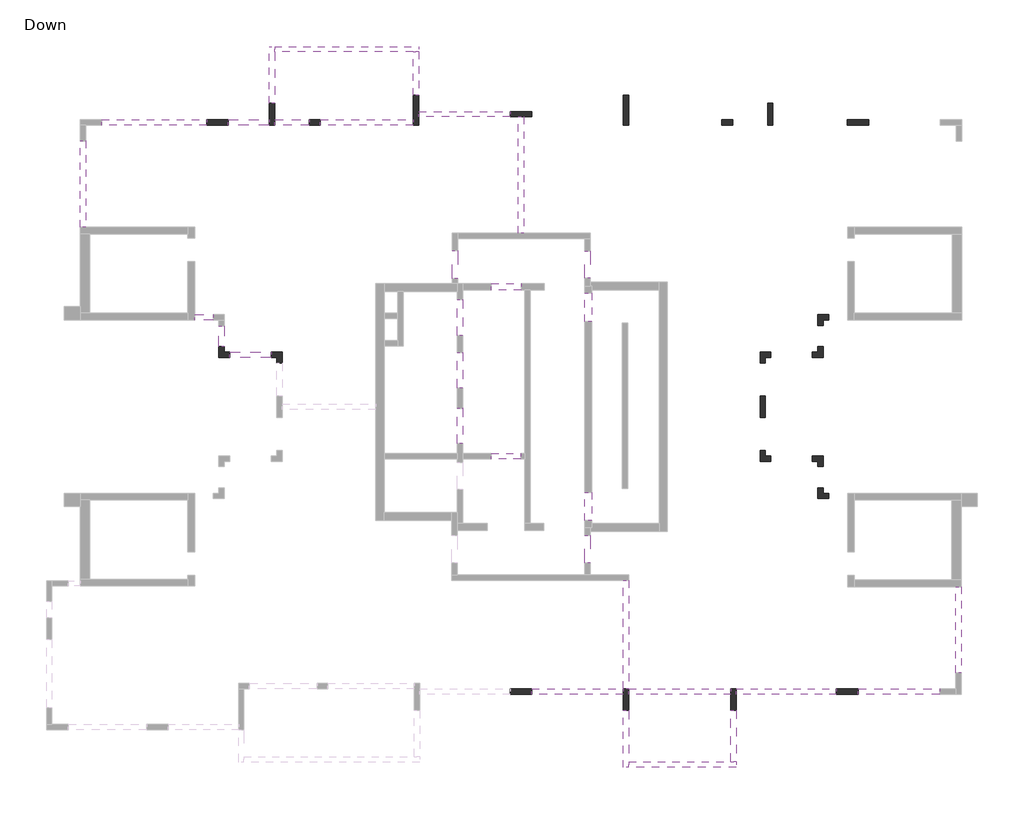
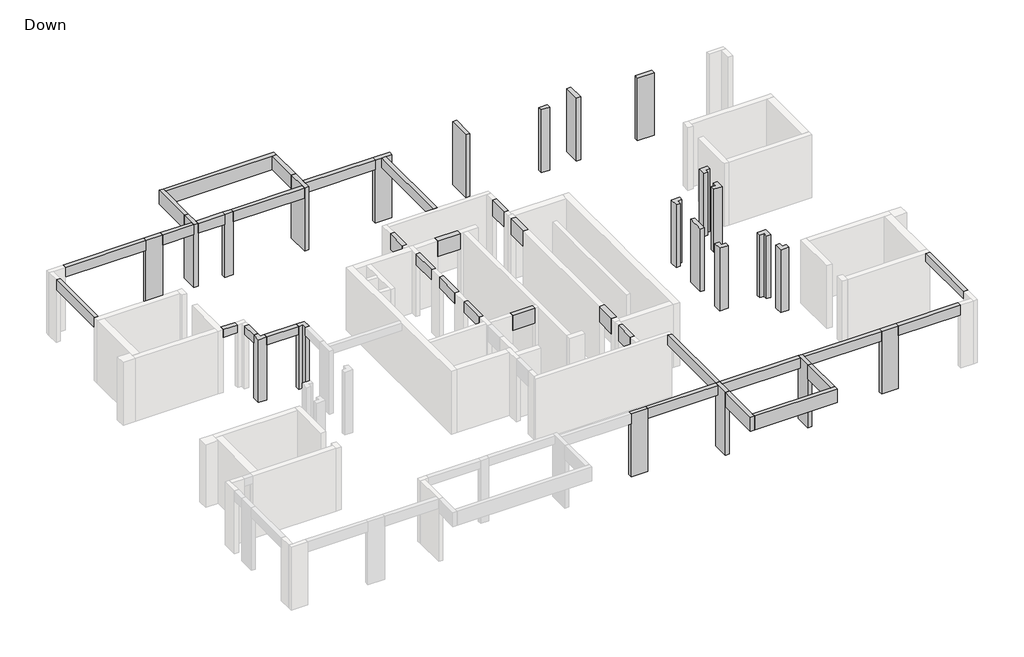
# One storey, part 3 of 3: 32 beams, 22 columns.
"""IFC4 building model written with IfcOpenShell, lengths in millimetres."""

from ifc_helpers import new_model, si_unit, frame, origin, origin_with_axes, place, context, project, spatial, polyline, outline, extrude, faceted_brep, element, save

model = new_model("IFC4")

# Units and contexts
model_context = context("Model", 3, world=origin())
ifc_project = project(units=[si_unit("LENGTHUNIT", "METRE", prefix="MILLI")], contexts=[model_context])

# Site, building, storey
site = spatial("IfcSite", under=ifc_project)
building = spatial("IfcBuilding", under=site)
storey = spatial("IfcBuildingStorey", under=building, Name="Down", Elevation=0.0)

# Beams
placement = place(None, origin())
element("IfcBeam", 1, ObjectType="Concrete Rectengular Beam : 20/40", at=placement, inside=storey, context=model_context, shape_type="Brep", body=[
    faceted_brep([(-11929.8186713, 1705.2784849, 3200.0), (-11929.8186713, 1505.2784849, 3200.0), (-11231.2965038, 1505.2784849, 3200.0), (-11231.2965038, 1705.2784849, 3200.0), (-11231.2965038, 1705.2784849, 3020.0), (-11231.2965038, 1705.2784849, 2800.0), (-11929.8186713, 1705.2784849, 2800.0), (-11929.8186713, 1705.2784849, 3020.0), (-11929.8186713, 1505.2784849, 2800.0), (-11231.2965038, 1505.2784849, 2800.0)], [[[0, 1, 2, 3]], [[0, 3, 4, 5, 6, 7]], [[8, 6, 5, 9]], [[1, 8, 9, 2]], [[1, 0, 7, 6, 8]], [[3, 2, 9, 5, 4]]]),
])
element("IfcBeam", 2, ObjectType="Concrete Rectengular Beam : 20/40", at=placement, inside=storey, context=model_context, shape_type="Brep", body=[
    faceted_brep([(-10831.2965038, 1285.2784849, 3200.0), (-11031.2965038, 1285.2784849, 3200.0), (-11031.2965038, 525.2784849, 3200.0), (-10831.2965038, 525.2784849, 3200.0), (-11031.2965038, 1285.2784849, 2800.0), (-11031.2965038, 525.2784849, 2800.0), (-10831.2965038, 1285.2784849, 2800.0), (-10831.2965038, 525.2784849, 2800.0), (-10831.2965038, 1285.2784849, 3020.0)], [[[0, 1, 2, 3]], [[1, 4, 5, 2]], [[4, 6, 7, 5]], [[6, 8, 0, 3, 7]], [[1, 0, 8, 6, 4]], [[3, 2, 5, 7]]]),
])
element("IfcBeam", 3, ObjectType="Concrete Rectengular Beam : 20/40", at=placement, inside=storey, context=model_context, shape_type="SweptSolid", body=[
    extrude(outline(polyline([(-10631.2965038, 125.2784849), (-10631.2965038, 325.2784849), (-9097.9894431, 325.2784849), (-9097.9894431, 125.2784849), (-10631.2965038, 125.2784849)])), frame((0.0, 0.0, 2800.0), z_axis=(0.0, 0.0, 1.0), x_axis=(1.0, 0.0, 0.0)), (0.0, 0.0, 1.0), 400.0),
])
element("IfcBeam", 4, ObjectType="Concrete Rectengular Beam : 20/40", at=placement, inside=storey, context=model_context, shape_type="Brep", body=[
    faceted_brep([(16390.4478267, -8347.5852261, 3200.0), (16190.4478267, -8347.5852261, 3200.0), (16190.4478267, -11524.2691374, 3200.0), (16390.4478267, -11524.2691374, 3200.0), (16390.4478267, -8347.5852261, 2800.0), (16390.4478267, -11524.2691374, 2800.0), (16190.4478267, -8347.5852261, 2800.0), (16190.4478267, -11524.2691374, 2800.0), (16190.4478267, -8347.5852261, 3020.0)], [[[0, 1, 2, 3]], [[4, 0, 3, 5]], [[6, 4, 5, 7]], [[1, 8, 6, 7, 2]], [[1, 0, 4, 6, 8]], [[3, 2, 7, 5]]]),
])
element("IfcBeam", 5, ObjectType="Concrete Rectengular Beam : 20/50", at=placement, inside=storey, context=model_context, shape_type="Brep", body=[
    faceted_brep([(-3849.7912929, 8714.1448811, 3200.0), (-3849.7912929, 8914.1448811, 3200.0), (-7285.8677257, 8914.1448811, 3200.0), (-7285.8677257, 8714.1448811, 3200.0), (-3849.7912929, 8914.1448811, 3020.0), (-3849.7912929, 8914.1448811, 2700.0), (-7285.8677257, 8914.1448811, 2700.0), (-3849.7912929, 8714.1448811, 2700.0), (-7285.8677257, 8714.1448811, 2700.0), (-7285.8677257, 8714.1448811, 3020.0), (-3849.7912929, 8714.1448811, 3020.0)], [[[0, 1, 2, 3]], [[1, 4, 5, 6, 2]], [[5, 7, 8, 6]], [[0, 3, 9, 8, 7, 10]], [[1, 0, 10, 7, 5, 4]], [[3, 2, 6, 8, 9]]]),
])
element("IfcBeam", 6, ObjectType="Concrete Rectengular Beam : 20/50", at=placement, inside=storey, context=model_context, shape_type="Brep", body=[
    faceted_brep([(-7685.8677257, 8714.1448811, 3200.0), (-7685.8677257, 8914.1448811, 3200.0), (-8975.1176117, 8914.1448811, 3200.0), (-8975.1176117, 8714.1448811, 3200.0), (-7685.8677257, 8914.1448811, 2700.0), (-8975.1176117, 8914.1448811, 2700.0), (-8975.1176117, 8914.1448811, 3020.0), (-7685.8677257, 8714.1448811, 2700.0), (-8975.1176117, 8714.1448811, 2700.0), (-8975.1176117, 8714.1448811, 3020.0), (-7685.8677257, 8714.1448811, 3020.0)], [[[0, 1, 2, 3]], [[1, 4, 5, 6, 2]], [[4, 7, 8, 5]], [[0, 3, 9, 8, 7, 10]], [[1, 0, 10, 7, 4]], [[3, 2, 6, 5, 8, 9]]]),
])
element("IfcBeam", 7, ObjectType="Concrete Rectengular Beam : 20/50", at=placement, inside=storey, context=model_context, shape_type="Brep", body=[
    faceted_brep([(-9175.1176117, 8714.1448811, 3200.0), (-9175.1176117, 8914.1448811, 3200.0), (-10684.1955166, 8914.1448811, 3200.0), (-10684.1955166, 8714.1448811, 3200.0), (-9175.1176117, 8914.1448811, 2700.0), (-10684.1955166, 8914.1448811, 2700.0), (-9175.1176117, 8714.1448811, 2700.0), (-10684.1955166, 8714.1448811, 2700.0), (-10684.1955166, 8714.1448811, 3020.0), (-9175.1176117, 8714.1448811, 3020.0)], [[[0, 1, 2, 3]], [[1, 4, 5, 2]], [[4, 6, 7, 5]], [[0, 3, 8, 7, 6, 9]], [[1, 0, 9, 6, 4]], [[3, 2, 5, 7, 8]]]),
])
element("IfcBeam", 8, ObjectType="Concrete Rectengular Beam : 20/50", at=placement, inside=storey, context=model_context, shape_type="Brep", body=[
    faceted_brep([(-11484.1955166, 8714.1448811, 3200.0), (-11484.1955166, 8914.1448811, 3200.0), (-15359.5625137, 8914.1448811, 3200.0), (-15359.5625137, 8714.1448811, 3200.0), (-11484.1955166, 8914.1448811, 2700.0), (-15359.5625137, 8914.1448811, 2700.0), (-11484.1955166, 8714.1448811, 2700.0), (-15359.5625137, 8714.1448811, 2700.0), (-15359.5625137, 8714.1448811, 3020.0), (-11484.1955166, 8714.1448811, 3020.0)], [[[0, 1, 2, 3]], [[1, 4, 5, 2]], [[4, 6, 7, 5]], [[0, 3, 8, 7, 6, 9]], [[1, 0, 9, 6, 4]], [[3, 2, 5, 7, 8]]]),
])
element("IfcBeam", 9, ObjectType="Concrete Rectengular Beam : 20/50", at=placement, inside=storey, context=model_context, shape_type="Brep", body=[
    faceted_brep([(-15952.3851738, 8125.9123109, 3200.0), (-16152.3851738, 8125.9123109, 3200.0), (-16152.3851738, 4939.6791417, 3200.0), (-15952.3851738, 4939.6791417, 3200.0), (-16152.3851738, 8125.9123109, 2700.0), (-16152.3851738, 4939.6791417, 2700.0), (-15952.3851738, 8125.9123109, 2700.0), (-15952.3851738, 4939.6791417, 2700.0), (-15952.3851738, 4939.6791417, 3020.0)], [[[0, 1, 2, 3]], [[1, 4, 5, 2]], [[4, 6, 7, 5]], [[6, 0, 3, 8, 7]], [[1, 0, 6, 4]], [[3, 2, 5, 7, 8]]]),
])
element("IfcBeam", 10, ObjectType="Concrete Rectengular Beam : 20/50", at=placement, inside=storey, context=model_context, shape_type="Brep", body=[
    faceted_brep([(-3649.7912929, 9214.1448811, 3200.0), (-3649.7912929, 9014.1448811, 3200.0), (-270.9686735, 9014.1448811, 3200.0), (-270.9686735, 9214.1448811, 3200.0), (-3649.7912929, 9214.1448811, 2700.0), (-270.9686735, 9214.1448811, 2700.0), (-3649.7912929, 9014.1448811, 2700.0), (-270.9686735, 9014.1448811, 2700.0), (-3649.7912929, 9014.1448811, 3020.0)], [[[0, 1, 2, 3]], [[4, 0, 3, 5]], [[6, 4, 5, 7]], [[1, 8, 6, 7, 2]], [[1, 0, 4, 6, 8]], [[3, 2, 7, 5]]]),
])
element("IfcBeam", 11, ObjectType="Concrete Rectengular Beam : 20/50", at=placement, inside=storey, context=model_context, shape_type="Brep", body=[
    faceted_brep([(229.0313265, 9014.1448811, 3200.0), (29.0313265, 9014.1448811, 3200.0), (29.0313265, 4709.9784533, 3200.0), (229.0313265, 4709.9784533, 3200.0), (29.0313265, 9014.1448811, 3020.0), (29.0313265, 9014.1448811, 2700.0), (29.0313265, 4709.9784533, 2700.0), (29.0313265, 4709.9784533, 3020.0), (229.0313265, 9014.1448811, 2700.0), (229.0313265, 4709.9784533, 2700.0), (229.0313265, 9014.1448811, 3020.0), (229.0313265, 4709.9784533, 3020.0)], [[[0, 1, 2, 3]], [[1, 4, 5, 6, 7, 2]], [[5, 8, 9, 6]], [[8, 10, 0, 3, 11, 9]], [[5, 4, 1, 0, 10, 8]], [[3, 2, 7, 6, 9, 11]]]),
])
element("IfcBeam", 12, ObjectType="Concrete Rectengular Beam : 20/50", at=placement, inside=storey, context=model_context, shape_type="SweptSolid", body=[
    extrude(outline(polyline([(12576.1675255, -12324.2691374), (12576.1675255, -12124.2691374), (15592.9268131, -12124.2691374), (15592.9268131, -12324.2691374), (12576.1675255, -12324.2691374)])), frame((0.0, 0.0, 2700.0), z_axis=(0.0, 0.0, 1.0), x_axis=(1.0, 0.0, 0.0)), (0.0, 0.0, 1.0), 500.0),
])
element("IfcBeam", 13, ObjectType="Concrete Rectengular Beam : 20/50", at=placement, inside=storey, context=model_context, shape_type="Brep", body=[
    faceted_brep([(11776.1675255, -12324.2691374, 3200.0), (11776.1675255, -12124.2691374, 3200.0), (8077.9664013, -12124.2691374, 3200.0), (8077.9664013, -12324.2691374, 3200.0), (11776.1675255, -12124.2691374, 2700.0), (8077.9664013, -12124.2691374, 2700.0), (8077.9664013, -12124.2691374, 3020.0), (11776.1675255, -12324.2691374, 2700.0), (8077.9664013, -12324.2691374, 2700.0)], [[[0, 1, 2, 3]], [[1, 4, 5, 6, 2]], [[4, 7, 8, 5]], [[7, 0, 3, 8]], [[1, 0, 7, 4]], [[3, 2, 6, 5, 8]]]),
])
element("IfcBeam", 14, ObjectType="Concrete Rectengular Beam : 20/50", at=placement, inside=storey, context=model_context, shape_type="Brep", body=[
    faceted_brep([(7877.9664013, -12324.2691374, 3200.0), (7877.9664013, -12124.2691374, 3200.0), (4107.8539459, -12124.2691374, 3200.0), (4107.8539459, -12324.2691374, 3200.0), (7877.9664013, -12124.2691374, 3020.0), (7877.9664013, -12124.2691374, 2700.0), (4107.8539459, -12124.2691374, 2700.0), (4107.8539459, -12124.2691374, 3020.0), (7877.9664013, -12324.2691374, 2700.0), (4107.8539459, -12324.2691374, 2700.0), (7877.9664013, -12324.2691374, 3020.0), (4107.8539459, -12324.2691374, 3020.0)], [[[0, 1, 2, 3]], [[1, 4, 5, 6, 7, 2]], [[5, 8, 9, 6]], [[8, 10, 0, 3, 11, 9]], [[1, 0, 10, 8, 5, 4]], [[3, 2, 7, 6, 9, 11]]]),
])
element("IfcBeam", 15, ObjectType="Concrete Rectengular Beam : 20/50", at=placement, inside=storey, context=model_context, shape_type="Brep", body=[
    faceted_brep([(3907.8539459, -12324.2691374, 3200.0), (3907.8539459, -12124.2691374, 3200.0), (529.0313265, -12124.2691374, 3200.0), (529.0313265, -12324.2691374, 3200.0), (3907.8539459, -12124.2691374, 3020.0), (3907.8539459, -12124.2691374, 2700.0), (529.0313265, -12124.2691374, 2700.0), (529.0313265, -12124.2691374, 3020.0), (3907.8539459, -12324.2691374, 2700.0), (529.0313265, -12324.2691374, 2700.0)], [[[0, 1, 2, 3]], [[2, 1, 4, 5, 6, 7]], [[5, 8, 9, 6]], [[8, 0, 3, 9]], [[1, 0, 8, 5, 4]], [[3, 2, 7, 6, 9]]]),
])
element("IfcBeam", 16, ObjectType="Concrete Rectengular Beam : 20/50", at=placement, inside=storey, context=model_context, shape_type="Brep", body=[
    faceted_brep([(3907.8539459, -12124.2691374, 3200.0), (4107.8539459, -12124.2691374, 3200.0), (4107.8539459, -8111.1752209, 3200.0), (3907.8539459, -8111.1752209, 3200.0), (4107.8539459, -12124.2691374, 3020.0), (4107.8539459, -12124.2691374, 2700.0), (4107.8539459, -8111.1752209, 2700.0), (3907.8539459, -12124.2691374, 2700.0), (3907.8539459, -8111.1752209, 2700.0), (3907.8539459, -12124.2691374, 3020.0), (3907.8539459, -8111.1752209, 3020.0)], [[[0, 1, 2, 3]], [[1, 4, 5, 6, 2]], [[5, 7, 8, 6]], [[7, 9, 0, 3, 10, 8]], [[0, 9, 7, 5, 4, 1]], [[3, 2, 6, 8, 10]]]),
])
element("IfcBeam", 17, ObjectType="Concrete Rectengular Beam : 20/53", at=placement, inside=storey, context=model_context, shape_type="SweptSolid", body=[
    extrude(outline(polyline([(3200.0, -2227.8189264), (2670.0, -2227.8189264), (2670.0, -2027.8189264), (3020.0, -2027.8189264), (3020.0, -2032.8189264), (3200.0, -2032.8189264), (3200.0, -2227.8189264)])), frame((0.0, 933.8247791, 0.0), z_axis=(0.0, 1.0, 0.0), x_axis=(0.0, 0.0, 1.0)), (0.0, 0.0, 1.0), 1325.0),
])
element("IfcBeam", 18, ObjectType="Concrete Rectengular Beam : 20/53", at=placement, inside=storey, context=model_context, shape_type="SweptSolid", body=[
    extrude(outline(polyline([(3200.0, -2227.8189264), (2670.0, -2227.8189264), (2670.0, -2027.8189264), (3020.0, -2027.8189264), (3020.0, -2032.8189264), (3200.0, -2032.8189264), (3200.0, -2227.8189264)])), frame((0.0, -1013.9530422, 0.0), z_axis=(0.0, 1.0, 0.0), x_axis=(0.0, 0.0, 1.0)), (0.0, 0.0, 1.0), 1327.7778213),
])
element("IfcBeam", 19, ObjectType="Concrete Rectengular Beam : 20/53", at=placement, inside=storey, context=model_context, shape_type="SweptSolid", body=[
    extrude(outline(polyline([(3200.0, -2227.8189264), (2670.0, -2227.8189264), (2670.0, -2027.8189264), (3020.0, -2027.8189264), (3020.0, -2032.8189264), (3200.0, -2032.8189264), (3200.0, -2227.8189264)])), frame((0.0, -3053.9530422, 0.0), z_axis=(0.0, 1.0, 0.0), x_axis=(0.0, 0.0, 1.0)), (0.0, 0.0, 1.0), 1300.0),
])
element("IfcBeam", 20, ObjectType="Concrete Rectengular Beam : 20/70", at=placement, inside=storey, context=model_context, shape_type="Brep", body=[
    faceted_brep([(-8975.1176117, 11614.1448811, 3200.0), (-9175.1176117, 11614.1448811, 3200.0), (-9175.1176117, 9514.1448811, 3200.0), (-8975.1176117, 9514.1448811, 3200.0), (-8975.1176117, 11414.1448811, 3200.0), (-8975.1176117, 11614.1448811, 2500.0), (-8975.1176117, 9514.1448811, 2500.0), (-8975.1176117, 11414.1448811, 2500.0), (-9175.1176117, 11614.1448811, 2500.0), (-9175.1176117, 9514.1448811, 2500.0)], [[[0, 1, 2, 3, 4]], [[5, 0, 4, 3, 6, 7]], [[8, 5, 7, 6, 9]], [[1, 8, 9, 2]], [[3, 2, 9, 6]], [[1, 0, 5, 8]]]),
])
element("IfcBeam", 21, ObjectType="Concrete Rectengular Beam : 20/70", at=placement, inside=storey, context=model_context, shape_type="Brep", body=[
    faceted_brep([(-3649.7912929, 11414.1448811, 3200.0), (-3649.7912929, 11614.1448811, 3200.0), (-8975.1176117, 11614.1448811, 3200.0), (-8975.1176117, 11414.1448811, 3200.0), (-3849.7912929, 11414.1448811, 3200.0), (-3649.7912929, 11414.1448811, 2500.0), (-8975.1176117, 11414.1448811, 3020.0), (-8975.1176117, 11414.1448811, 2500.0), (-3849.7912929, 11414.1448811, 2500.0), (-3649.7912929, 11614.1448811, 2500.0), (-8975.1176117, 11614.1448811, 2500.0)], [[[0, 1, 2, 3, 4]], [[5, 0, 4, 3, 6, 7, 8]], [[9, 5, 8, 7, 10]], [[1, 9, 10, 2]], [[3, 2, 10, 7, 6]], [[1, 0, 5, 9]]]),
])
element("IfcBeam", 22, ObjectType="Concrete Rectengular Beam : 20/70", at=placement, inside=storey, context=model_context, shape_type="Brep", body=[
    faceted_brep([(-3849.7912929, 9814.1448811, 3200.0), (-3649.7912929, 9814.1448811, 3200.0), (-3649.7912929, 11414.1448811, 3200.0), (-3849.7912929, 11414.1448811, 3200.0), (-3849.7912929, 9814.1448811, 2500.0), (-3849.7912929, 11414.1448811, 3020.0), (-3849.7912929, 11414.1448811, 2500.0), (-3649.7912929, 9814.1448811, 2500.0), (-3649.7912929, 11414.1448811, 2500.0)], [[[0, 1, 2, 3]], [[4, 0, 3, 5, 6]], [[7, 4, 6, 8]], [[1, 7, 8, 2]], [[1, 0, 4, 7]], [[3, 2, 8, 6, 5]]]),
])
element("IfcBeam", 23, ObjectType="Concrete Rectengular Beam : 20/70", at=placement, inside=storey, context=model_context, shape_type="Brep", body=[
    faceted_brep([(3907.8539459, -15024.2691374, 3200.0), (4107.8539459, -15024.2691374, 3200.0), (4107.8539459, -14824.2691374, 3200.0), (4107.8539459, -12924.2691374, 3200.0), (3907.8539459, -12924.2691374, 3200.0), (3907.8539459, -15024.2691374, 2500.0), (3907.8539459, -12924.2691374, 2500.0), (4107.8539459, -15024.2691374, 2500.0), (4107.8539459, -12924.2691374, 2500.0), (4107.8539459, -14824.2691374, 2500.0)], [[[0, 1, 2, 3, 4]], [[5, 0, 4, 6]], [[7, 5, 6, 8, 9]], [[1, 7, 9, 8, 3, 2]], [[4, 3, 8, 6]], [[1, 0, 5, 7]]]),
])
element("IfcBeam", 24, ObjectType="Concrete Rectengular Beam : 20/70", at=placement, inside=storey, context=model_context, shape_type="Brep", body=[
    faceted_brep([(8077.9664013, -15024.2691374, 3200.0), (8077.9664013, -14824.2691374, 3200.0), (7877.9664013, -14824.2691374, 3200.0), (4107.8539459, -14824.2691374, 3200.0), (4107.8539459, -15024.2691374, 3200.0), (8077.9664013, -15024.2691374, 2500.0), (4107.8539459, -15024.2691374, 2500.0), (8077.9664013, -14824.2691374, 2500.0), (4107.8539459, -14824.2691374, 2500.0), (7877.9664013, -14824.2691374, 2500.0), (4107.8539459, -14824.2691374, 3020.0)], [[[0, 1, 2, 3, 4]], [[5, 0, 4, 6]], [[7, 5, 6, 8, 9]], [[1, 7, 9, 8, 10, 3, 2]], [[4, 3, 10, 8, 6]], [[1, 0, 5, 7]]]),
])
element("IfcBeam", 25, ObjectType="Concrete Rectengular Beam : 20/70", at=placement, inside=storey, context=model_context, shape_type="Brep", body=[
    faceted_brep([(8077.9664013, -12920.4851141, 3200.0), (7877.9664013, -12920.4851141, 3200.0), (7877.9664013, -14824.2691374, 3200.0), (8077.9664013, -14824.2691374, 3200.0), (8077.9664013, -12920.4851141, 2500.0), (8077.9664013, -14824.2691374, 2500.0), (7877.9664013, -12920.4851141, 2500.0), (7877.9664013, -14824.2691374, 2500.0), (7877.9664013, -14824.2691374, 3020.0)], [[[0, 1, 2, 3]], [[4, 0, 3, 5]], [[6, 4, 5, 7]], [[1, 6, 7, 8, 2]], [[1, 0, 4, 6]], [[3, 2, 8, 7, 5]]]),
])
element("IfcBeam", 26, ObjectType="Concrete Rectengular Beam : 20/78", at=placement, inside=storey, context=model_context, shape_type="Brep", body=[
    faceted_brep([(-2415.274667, 3043.8247791, 3200.0), (-2215.274667, 3043.8247791, 3200.0), (-2215.274667, 4069.9784533, 3200.0), (-2415.274667, 4069.9784533, 3200.0), (-2215.274667, 3043.8247791, 3020.0), (-2215.274667, 3043.8247791, 2420.0), (-2215.274667, 4069.9784533, 2420.0), (-2215.274667, 4069.9784533, 3020.0), (-2415.274667, 3043.8247791, 2420.0), (-2415.274667, 4069.9784533, 2420.0), (-2415.274667, 4069.9784533, 3020.0), (-2415.274667, 3043.8247791, 3020.0)], [[[0, 1, 2, 3]], [[2, 1, 4, 5, 6, 7]], [[5, 8, 9, 6]], [[0, 3, 10, 9, 8, 11]], [[1, 0, 11, 8, 5, 4]], [[3, 2, 7, 6, 9, 10]]]),
])
element("IfcBeam", 27, ObjectType="Concrete Rectengular Beam : 20/78", at=placement, inside=storey, context=model_context, shape_type="SweptSolid", body=[
    extrude(outline(polyline([(2484.725333, 4049.9784533), (2684.725333, 4049.9784533), (2684.725333, 3056.2932633), (2484.725333, 3056.2932633), (2484.725333, 4049.9784533)])), frame((0.0, 0.0, 2420.0), z_axis=(0.0, 0.0, 1.0), x_axis=(1.0, 0.0, 0.0)), (0.0, 0.0, 1.0), 780.0),
])
element("IfcBeam", 28, ObjectType="Concrete Rectengular Beam : 20/78", at=placement, inside=storey, context=model_context, shape_type="Brep", body=[
    faceted_brep([(-967.8189264, -3433.9530422, 3200.0), (-967.8189264, -3433.9530422, 2420.0), (-967.8189264, -3633.9530422, 2420.0), (-967.8189264, -3633.9530422, 3020.0), (-967.8189264, -3633.9530422, 3200.0), (122.0171251, -3633.9530422, 3200.0), (122.0171251, -3433.9530422, 3200.0), (122.0171251, -3633.9530422, 2420.0), (122.0171251, -3633.9530422, 3020.0), (122.0171251, -3433.9530422, 2420.0)], [[[0, 1, 2, 3, 4]], [[0, 4, 5, 6]], [[5, 4, 3, 2, 7, 8]], [[2, 1, 9, 7]], [[1, 0, 6, 9]], [[6, 5, 8, 7, 9]]]),
])
element("IfcBeam", 29, ObjectType="Concrete Rectengular Beam : 20/78", at=placement, inside=storey, context=model_context, shape_type="SweptSolid", body=[
    extrude(outline(polyline([(2484.725333, -6451.1752209), (2684.725333, -6451.1752209), (2684.725333, -7471.1752209), (2484.725333, -7471.1752209), (2484.725333, -6451.1752209)])), frame((0.0, 0.0, 2420.0), z_axis=(0.0, 0.0, 1.0), x_axis=(1.0, 0.0, 0.0)), (0.0, 0.0, 1.0), 780.0),
])
element("IfcBeam", 30, ObjectType="Concrete Rectengular Beam : 25/78", at=placement, inside=storey, context=model_context, shape_type="Brep", body=[
    faceted_brep([(-972.8189264, 2858.8247791, 3200.0), (-972.8189264, 2608.8247791, 3200.0), (132.1810736, 2608.8247791, 3200.0), (132.1810736, 2858.8247791, 3200.0), (-972.8189264, 2608.8247791, 2420.0), (132.1810736, 2608.8247791, 2420.0), (-972.8189264, 2858.8247791, 2420.0), (132.1810736, 2858.8247791, 2420.0), (132.1810736, 2858.8247791, 3020.0), (-972.8189264, 2858.8247791, 3020.0)], [[[0, 1, 2, 3]], [[1, 4, 5, 2]], [[4, 6, 7, 5]], [[0, 3, 8, 7, 6, 9]], [[1, 0, 9, 6, 4]], [[3, 2, 5, 7, 8]]]),
])
element("IfcBeam", 31, ObjectType="Concrete Rectengular Beam : 25/78", at=placement, inside=storey, context=model_context, shape_type="SweptSolid", body=[
    extrude(outline(polyline([(2484.725333, 2496.2932633), (2734.725333, 2496.2932633), (2734.725333, 1454.2743435), (2484.725333, 1454.2743435), (2484.725333, 2496.2932633)])), frame((0.0, 0.0, 2420.0), z_axis=(0.0, 0.0, 1.0), x_axis=(1.0, 0.0, 0.0)), (0.0, 0.0, 1.0), 780.0),
])
element("IfcBeam", 32, ObjectType="Concrete Rectengular Beam : 25/78", at=placement, inside=storey, context=model_context, shape_type="SweptSolid", body=[
    extrude(outline(polyline([(2734.725333, -5901.1752209), (2484.725333, -5901.1752209), (2484.725333, -4865.7256565), (2734.725333, -4865.7256565), (2734.725333, -5901.1752209)])), frame((0.0, 0.0, 2420.0), z_axis=(0.0, 0.0, 1.0), x_axis=(1.0, 0.0, 0.0)), (0.0, 0.0, 1.0), 780.0),
])

# Columns
element("IfcColumn", 33, ObjectType="Concrete Rectengular Column : 20/110", at=placement, inside=storey, context=model_context, shape_type="Brep", body=[
    faceted_brep([(-3649.7912929, 9814.1448811, 0.0), (-3649.7912929, 8714.1448811, 0.0), (-3849.7912929, 8714.1448811, 0.0), (-3849.7912929, 9814.1448811, 0.0), (-3649.7912929, 9814.1448811, 3200.0), (-3649.7912929, 9014.1448811, 3200.0), (-3649.7912929, 8714.1448811, 3200.0), (-3649.7912929, 8714.1448811, 3020.0), (-3849.7912929, 8714.1448811, 3200.0), (-3849.7912929, 8914.1448811, 3200.0), (-3849.7912929, 9814.1448811, 3200.0)], [[[0, 1, 2, 3]], [[4, 5, 6, 7, 1, 0]], [[6, 8, 2, 1, 7]], [[8, 9, 10, 3, 2]], [[10, 4, 0, 3]], [[4, 10, 9, 8, 6, 5]]]),
])
element("IfcColumn", 34, ObjectType="Concrete Rectengular Column : 20/110", at=placement, inside=storey, context=model_context, shape_type="Brep", body=[
    faceted_brep([(3907.8539459, 9814.1448811, 0.0), (4107.8539459, 9814.1448811, 0.0), (4107.8539459, 8714.1448811, 0.0), (3907.8539459, 8714.1448811, 0.0), (3907.8539459, 9814.1448811, 3200.0), (3907.8539459, 8714.1448811, 3020.0), (3907.8539459, 8714.1448811, 3200.0), (3907.8539459, 9014.1448811, 3200.0), (4107.8539459, 8714.1448811, 3200.0), (4107.8539459, 9814.1448811, 3200.0), (4107.8539459, 8914.1448811, 3200.0)], [[[0, 1, 2, 3]], [[4, 0, 3, 5, 6, 7]], [[6, 5, 3, 2, 8]], [[8, 2, 1, 9, 10]], [[9, 1, 0, 4]], [[4, 7, 6, 8, 10, 9]]]),
])
element("IfcColumn", 35, ObjectType="Concrete Rectengular Column : 20/40", at=placement, inside=storey, context=model_context, shape_type="SweptSolid", body=[
    extrude(outline(polyline([(-7685.8677257, 8914.1448811), (-7285.8677257, 8914.1448811), (-7285.8677257, 8714.1448811), (-7685.8677257, 8714.1448811), (-7685.8677257, 8914.1448811)])), origin_with_axes(), (0.0, 0.0, 1.0), 3200.0),
])
element("IfcColumn", 36, ObjectType="Concrete Rectengular Column : 20/40", at=placement, inside=storey, context=model_context, shape_type="SweptSolid", body=[
    extrude(outline(polyline([(7943.9303787, 8914.1448811), (7943.9303787, 8714.1448811), (7543.9303787, 8714.1448811), (7543.9303787, 8914.1448811), (7943.9303787, 8914.1448811)])), origin_with_axes(), (0.0, 0.0, 1.0), 3200.0),
])
element("IfcColumn", 37, ObjectType="Concrete Rectengular Column : 20/80", at=placement, inside=storey, context=model_context, shape_type="Brep", body=[
    faceted_brep([(-8975.1176117, 9514.1448811, 0.0), (-8975.1176117, 8714.1448811, 0.0), (-9175.1176117, 8714.1448811, 0.0), (-9175.1176117, 9514.1448811, 0.0), (-8975.1176117, 9514.1448811, 3200.0), (-8975.1176117, 8914.1448811, 3200.0), (-8975.1176117, 8714.1448811, 3200.0), (-9175.1176117, 8714.1448811, 3200.0), (-9175.1176117, 9514.1448811, 3200.0)], [[[0, 1, 2, 3]], [[4, 5, 6, 1, 0]], [[6, 7, 2, 1]], [[7, 8, 3, 2]], [[8, 4, 0, 3]], [[4, 8, 7, 6, 5]]]),
])
element("IfcColumn", 38, ObjectType="Concrete Rectengular Column : 20/80", at=placement, inside=storey, context=model_context, shape_type="SweptSolid", body=[
    extrude(outline(polyline([(-11484.1955166, 8914.1448811), (-10684.1955166, 8914.1448811), (-10684.1955166, 8714.1448811), (-11484.1955166, 8714.1448811), (-11484.1955166, 8914.1448811)])), origin_with_axes(), (0.0, 0.0, 1.0), 3200.0),
])
element("IfcColumn", 39, ObjectType="Concrete Rectengular Column : 20/80", at=placement, inside=storey, context=model_context, shape_type="Brep", body=[
    faceted_brep([(-270.9686735, 9214.1448811, 0.0), (529.0313265, 9214.1448811, 0.0), (529.0313265, 9014.1448811, 0.0), (-270.9686735, 9014.1448811, 0.0), (-270.9686735, 9214.1448811, 3200.0), (529.0313265, 9214.1448811, 3200.0), (529.0313265, 9014.1448811, 3200.0), (229.0313265, 9014.1448811, 3200.0), (29.0313265, 9014.1448811, 3200.0), (-270.9686735, 9014.1448811, 3200.0)], [[[0, 1, 2, 3]], [[4, 5, 1, 0]], [[5, 6, 2, 1]], [[6, 7, 8, 9, 3, 2]], [[9, 4, 0, 3]], [[4, 9, 8, 7, 6, 5]]]),
])
element("IfcColumn", 40, ObjectType="Concrete Rectengular Column : 20/80", at=placement, inside=storey, context=model_context, shape_type="Brep", body=[
    faceted_brep([(9233.1802646, 9514.1448811, 0.0), (9433.1802646, 9514.1448811, 0.0), (9433.1802646, 8714.1448811, 0.0), (9233.1802646, 8714.1448811, 0.0), (9233.1802646, 9514.1448811, 3200.0), (9233.1802646, 8714.1448811, 3200.0), (9233.1802646, 8914.1448811, 3200.0), (9433.1802646, 8714.1448811, 3200.0), (9433.1802646, 9514.1448811, 3200.0)], [[[0, 1, 2, 3]], [[4, 0, 3, 5, 6]], [[5, 3, 2, 7]], [[7, 2, 1, 8]], [[8, 1, 0, 4]], [[4, 6, 5, 7, 8]]]),
])
element("IfcColumn", 41, ObjectType="Concrete Rectengular Column : 20/80", at=placement, inside=storey, context=model_context, shape_type="SweptSolid", body=[
    extrude(outline(polyline([(12972.2581695, 8914.1448811), (12972.2581695, 8714.1448811), (12172.2581695, 8714.1448811), (12172.2581695, 8914.1448811), (12972.2581695, 8914.1448811)])), origin_with_axes(), (0.0, 0.0, 1.0), 3200.0),
])
element("IfcColumn", 42, ObjectType="Concrete Rectengular Column : 20/80", at=placement, inside=storey, context=model_context, shape_type="Brep", body=[
    faceted_brep([(8956.052096, -1293.9530422, 0.0), (9156.052096, -1293.9530422, 0.0), (9156.052096, -2093.9530422, 0.0), (8956.052096, -2093.9530422, 0.0), (8956.052096, -1293.9530422, 3200.0), (8956.052096, -1293.9530422, 2800.0), (8956.052096, -2093.9530422, 3200.0), (8956.052096, -1793.9530422, 3200.0), (8956.052096, -1593.9530422, 3200.0), (9156.052096, -2093.9530422, 3200.0), (9156.052096, -1293.9530422, 2800.0), (9156.052096, -1293.9530422, 3200.0)], [[[0, 1, 2, 3]], [[4, 5, 0, 3, 6, 7, 8]], [[6, 3, 2, 9]], [[9, 2, 1, 10, 11]], [[11, 10, 1, 0, 5, 4]], [[4, 8, 7, 6, 9, 11]]]),
])
element("IfcColumn", 43, ObjectType="Concrete Rectengular Column : 20/80", at=placement, inside=storey, context=model_context, shape_type="SweptSolid", body=[
    extrude(outline(polyline([(11776.1675255, -12124.2691374), (12576.1675255, -12124.2691374), (12576.1675255, -12324.2691374), (11776.1675255, -12324.2691374), (11776.1675255, -12124.2691374)])), origin_with_axes(), (0.0, 0.0, 1.0), 3200.0),
])
element("IfcColumn", 44, ObjectType="Concrete Rectengular Column : 20/80", at=placement, inside=storey, context=model_context, shape_type="Brep", body=[
    faceted_brep([(8077.9664013, -12120.4851141, 0.0), (8077.9664013, -12920.4851141, 0.0), (7877.9664013, -12920.4851141, 0.0), (7877.9664013, -12120.4851141, 0.0), (8077.9664013, -12120.4851141, 3200.0), (8077.9664013, -12124.2691374, 3200.0), (8077.9664013, -12920.4851141, 3200.0), (8077.9664013, -12120.4851141, 3020.0), (7877.9664013, -12920.4851141, 3200.0), (7877.9664013, -12324.2691374, 3200.0), (7877.9664013, -12124.2691374, 3200.0), (7877.9664013, -12120.4851141, 3200.0), (7877.9664013, -12120.4851141, 3020.0)], [[[0, 1, 2, 3]], [[4, 5, 6, 1, 0, 7]], [[6, 8, 2, 1]], [[8, 9, 10, 11, 12, 3, 2]], [[11, 4, 7, 0, 3, 12]], [[4, 11, 10, 9, 8, 6, 5]]]),
])
element("IfcColumn", 45, ObjectType="Concrete Rectengular Column : 20/80", at=placement, inside=storey, context=model_context, shape_type="Brep", body=[
    faceted_brep([(4107.8539459, -12124.2691374, 0.0), (4107.8539459, -12924.2691374, 0.0), (3907.8539459, -12924.2691374, 0.0), (3907.8539459, -12124.2691374, 0.0), (4107.8539459, -12124.2691374, 3200.0), (4107.8539459, -12324.2691374, 3200.0), (4107.8539459, -12924.2691374, 3200.0), (3907.8539459, -12924.2691374, 3200.0), (3907.8539459, -12124.2691374, 3200.0)], [[[0, 1, 2, 3]], [[4, 5, 6, 1, 0]], [[6, 7, 2, 1]], [[7, 8, 3, 2]], [[8, 4, 0, 3]], [[4, 8, 7, 6, 5]]]),
])
element("IfcColumn", 46, ObjectType="Concrete Rectengular Column : 20/80", at=placement, inside=storey, context=model_context, shape_type="SweptSolid", body=[
    extrude(outline(polyline([(-270.9686735, -12124.2691374), (529.0313265, -12124.2691374), (529.0313265, -12324.2691374), (-270.9686735, -12324.2691374), (-270.9686735, -12124.2691374)])), origin_with_axes(), (0.0, 0.0, 1.0), 3200.0),
])
element("IfcColumn", 47, ObjectType="L Column : 40/40/20/20", at=placement, inside=storey, context=model_context, shape_type="Brep", body=[
    faceted_brep([(-11031.2965038, 125.2784849, 0.0), (-11031.2965038, 525.2784849, 0.0), (-10831.2965038, 525.2784849, 0.0), (-10831.2965038, 325.2784849, 0.0), (-10631.2965038, 325.2784849, 0.0), (-10631.2965038, 125.2784849, 0.0), (-11031.2965038, 125.2784849, 3200.0), (-11031.2965038, 525.2784849, 3200.0), (-11031.2965038, 525.2784849, 2800.0), (-10831.2965038, 525.2784849, 3200.0), (-10831.2965038, 525.2784849, 2800.0), (-10831.2965038, 325.2784849, 3200.0), (-10831.2965038, 325.2784849, 3020.0), (-10631.2965038, 325.2784849, 3200.0), (-10631.2965038, 325.2784849, 2800.0), (-10631.2965038, 125.2784849, 3200.0), (-10631.2965038, 125.2784849, 2800.0)], [[[0, 1, 2, 3, 4, 5]], [[6, 7, 8, 1, 0]], [[7, 9, 10, 2, 1, 8]], [[9, 11, 12, 3, 2, 10]], [[11, 13, 14, 4, 3, 12]], [[13, 15, 16, 5, 4, 14]], [[15, 6, 0, 5, 16]], [[6, 15, 13, 11, 9, 7]]]),
])
element("IfcColumn", 48, ObjectType="L Column : 40/40/20/20", at=placement, inside=storey, context=model_context, shape_type="Brep", body=[
    faceted_brep([(-8697.9894431, 325.2784849, 0.0), (-8697.9894431, -74.7215151, 0.0), (-8897.9894431, -74.7215151, 0.0), (-8897.9894431, 125.2784849, 0.0), (-9097.9894431, 125.2784849, 0.0), (-9097.9894431, 325.2784849, 0.0), (-8697.9894431, 325.2784849, 3200.0), (-8697.9894431, -74.7215151, 3200.0), (-8697.9894431, -74.7215151, 2800.0), (-8697.9894431, 325.2784849, 3020.0), (-8897.9894431, -74.7215151, 3200.0), (-8897.9894431, -74.7215151, 2800.0), (-8897.9894431, 125.2784849, 3200.0), (-9097.9894431, 125.2784849, 3200.0), (-9097.9894431, 125.2784849, 2800.0), (-9097.9894431, 325.2784849, 3200.0), (-9097.9894431, 325.2784849, 2800.0)], [[[0, 1, 2, 3, 4, 5]], [[6, 7, 8, 1, 0, 9]], [[7, 10, 11, 2, 1, 8]], [[10, 12, 3, 2, 11]], [[12, 13, 14, 4, 3]], [[13, 15, 16, 5, 4, 14]], [[15, 6, 9, 0, 5, 16]], [[6, 15, 13, 12, 10, 7]]]),
])
element("IfcColumn", 49, ObjectType="L Column : 40/40/20/20", at=placement, inside=storey, context=model_context, shape_type="Brep", body=[
    faceted_brep([(11089.3591568, -5093.1845693, 0.0), (11089.3591568, -4693.1845693, 0.0), (11289.3591568, -4693.1845693, 0.0), (11289.3591568, -4893.1845693, 0.0), (11489.3591568, -4893.1845693, 0.0), (11489.3591568, -5093.1845693, 0.0), (11089.3591568, -5093.1845693, 3200.0), (11089.3591568, -4693.1845693, 3200.0), (11089.3591568, -4693.1845693, 2800.0), (11089.3591568, -5093.1845693, 3020.0), (11289.3591568, -4693.1845693, 3200.0), (11289.3591568, -4693.1845693, 2800.0), (11289.3591568, -4893.1845693, 3200.0), (11489.3591568, -4893.1845693, 3200.0), (11489.3591568, -4893.1845693, 2800.0), (11489.3591568, -5093.1845693, 3200.0), (11489.3591568, -5093.1845693, 2800.0)], [[[0, 1, 2, 3, 4, 5]], [[6, 7, 8, 1, 0, 9]], [[7, 10, 11, 2, 1, 8]], [[10, 12, 3, 2, 11]], [[12, 13, 14, 4, 3]], [[13, 15, 16, 5, 4, 14]], [[15, 6, 9, 0, 5, 16]], [[6, 15, 13, 12, 10, 7]]]),
])
element("IfcColumn", 50, ObjectType="L Column : 40/40/20/20", at=placement, inside=storey, context=model_context, shape_type="Brep", body=[
    faceted_brep([(11289.3591568, -3513.1845693, 0.0), (11289.3591568, -3913.1845693, 0.0), (11089.3591568, -3913.1845693, 0.0), (11089.3591568, -3713.1845693, 0.0), (10889.3591568, -3713.1845693, 0.0), (10889.3591568, -3513.1845693, 0.0), (11289.3591568, -3513.1845693, 3200.0), (11289.3591568, -3913.1845693, 3200.0), (11289.3591568, -3913.1845693, 2800.0), (11089.3591568, -3913.1845693, 3200.0), (11089.3591568, -3913.1845693, 2800.0), (11089.3591568, -3713.1845693, 3200.0), (11089.3591568, -3713.1845693, 3020.0), (10889.3591568, -3713.1845693, 3200.0), (10889.3591568, -3713.1845693, 2800.0), (10889.3591568, -3513.1845693, 3200.0), (10889.3591568, -3513.1845693, 2800.0)], [[[0, 1, 2, 3, 4, 5]], [[6, 7, 8, 1, 0]], [[7, 9, 10, 2, 1, 8]], [[9, 11, 12, 3, 2, 10]], [[11, 13, 14, 4, 3, 12]], [[13, 15, 16, 5, 4, 14]], [[15, 6, 0, 5, 16]], [[6, 15, 13, 11, 9, 7]]]),
])
element("IfcColumn", 51, ObjectType="L Column : 40/40/20/20", at=placement, inside=storey, context=model_context, shape_type="Brep", body=[
    faceted_brep([(8956.052096, -3713.1845693, 0.0), (8956.052096, -3313.1845693, 0.0), (9156.052096, -3313.1845693, 0.0), (9156.052096, -3513.1845693, 0.0), (9356.052096, -3513.1845693, 0.0), (9356.052096, -3713.1845693, 0.0), (8956.052096, -3713.1845693, 3200.0), (8956.052096, -3313.1845693, 3200.0), (8956.052096, -3313.1845693, 2800.0), (8956.052096, -3713.1845693, 3020.0), (9156.052096, -3313.1845693, 3200.0), (9156.052096, -3313.1845693, 2800.0), (9156.052096, -3513.1845693, 3200.0), (9356.052096, -3513.1845693, 3200.0), (9356.052096, -3513.1845693, 2800.0), (9356.052096, -3713.1845693, 3200.0), (9356.052096, -3713.1845693, 2800.0)], [[[0, 1, 2, 3, 4, 5]], [[6, 7, 8, 1, 0, 9]], [[7, 10, 11, 2, 1, 8]], [[10, 12, 3, 2, 11]], [[12, 13, 14, 4, 3]], [[13, 15, 16, 5, 4, 14]], [[15, 6, 9, 0, 5, 16]], [[6, 15, 13, 12, 10, 7]]]),
])
element("IfcColumn", 52, ObjectType="L Column : 40/40/20/20", at=placement, inside=storey, context=model_context, shape_type="Brep", body=[
    faceted_brep([(8956.052096, 325.2784849, 0.0), (9356.052096, 325.2784849, 0.0), (9356.052096, 125.2784849, 0.0), (9156.052096, 125.2784849, 0.0), (9156.052096, -74.7215151, 0.0), (8956.052096, -74.7215151, 0.0), (8956.052096, 325.2784849, 3200.0), (9356.052096, 325.2784849, 3200.0), (9356.052096, 325.2784849, 2800.0), (8956.052096, 325.2784849, 3020.0), (9356.052096, 125.2784849, 3200.0), (9356.052096, 125.2784849, 2800.0), (9156.052096, 125.2784849, 3200.0), (9156.052096, -74.7215151, 3200.0), (9156.052096, -74.7215151, 2800.0), (8956.052096, -74.7215151, 3200.0), (8956.052096, -74.7215151, 2800.0)], [[[0, 1, 2, 3, 4, 5]], [[6, 7, 8, 1, 0, 9]], [[7, 10, 11, 2, 1, 8]], [[10, 12, 3, 2, 11]], [[12, 13, 14, 4, 3]], [[13, 15, 16, 5, 4, 14]], [[15, 6, 9, 0, 5, 16]], [[6, 15, 13, 12, 10, 7]]]),
])
element("IfcColumn", 53, ObjectType="L Column : 40/40/20/20", at=placement, inside=storey, context=model_context, shape_type="Brep", body=[
    faceted_brep([(11289.3591568, 125.2784849, 0.0), (10889.3591568, 125.2784849, 0.0), (10889.3591568, 325.2784849, 0.0), (11089.3591568, 325.2784849, 0.0), (11089.3591568, 525.2784849, 0.0), (11289.3591568, 525.2784849, 0.0), (11289.3591568, 125.2784849, 3200.0), (10889.3591568, 125.2784849, 3200.0), (10889.3591568, 125.2784849, 2800.0), (10889.3591568, 325.2784849, 3200.0), (10889.3591568, 325.2784849, 2800.0), (11089.3591568, 325.2784849, 3200.0), (11089.3591568, 325.2784849, 3020.0), (11089.3591568, 525.2784849, 3200.0), (11089.3591568, 525.2784849, 2800.0), (11289.3591568, 525.2784849, 3200.0), (11289.3591568, 525.2784849, 2800.0)], [[[0, 1, 2, 3, 4, 5]], [[6, 7, 8, 1, 0]], [[7, 9, 10, 2, 1, 8]], [[9, 11, 12, 3, 2, 10]], [[11, 13, 14, 4, 3, 12]], [[13, 15, 16, 5, 4, 14]], [[15, 6, 0, 5, 16]], [[6, 15, 13, 11, 9, 7]]]),
])
element("IfcColumn", 54, ObjectType="L Column : 40/40/20/20", at=placement, inside=storey, context=model_context, shape_type="Brep", body=[
    faceted_brep([(11089.3591568, 1705.2784849, 0.0), (11489.3591568, 1705.2784849, 0.0), (11489.3591568, 1505.2784849, 0.0), (11289.3591568, 1505.2784849, 0.0), (11289.3591568, 1305.2784849, 0.0), (11089.3591568, 1305.2784849, 0.0), (11089.3591568, 1705.2784849, 3200.0), (11489.3591568, 1705.2784849, 3200.0), (11489.3591568, 1705.2784849, 2800.0), (11089.3591568, 1705.2784849, 3020.0), (11489.3591568, 1505.2784849, 3200.0), (11489.3591568, 1505.2784849, 2800.0), (11289.3591568, 1505.2784849, 3200.0), (11289.3591568, 1305.2784849, 3200.0), (11289.3591568, 1305.2784849, 2800.0), (11089.3591568, 1305.2784849, 3200.0), (11089.3591568, 1305.2784849, 2800.0)], [[[0, 1, 2, 3, 4, 5]], [[6, 7, 8, 1, 0, 9]], [[7, 10, 11, 2, 1, 8]], [[10, 12, 3, 2, 11]], [[12, 13, 14, 4, 3]], [[13, 15, 16, 5, 4, 14]], [[15, 6, 9, 0, 5, 16]], [[6, 15, 13, 12, 10, 7]]]),
])

save(model, "model.ifc")

# Revit data of these elements
# Type "Concrete Rectengular Beam : 20/40"
#   Keynote = "09000"
#   Length [instance default] = 152.4 cm
#   b = 20 cm
#   h = 40 cm
#   Structural Material [instance default] = Concrete
#   Assembly Code = ""
# Type "Concrete Rectengular Beam : 20/50"
#   Length [instance default] = 152.4 cm
#   b = 20 cm
#   h = 50 cm
#   Structural Material [instance default] = Concrete
#   Assembly Code = ""
# Type "Concrete Rectengular Beam : 20/53"
#   Length [instance default] = 152.4 cm
#   b = 20 cm
#   h = 53 cm
#   Structural Material [instance default] = Concrete
#   Assembly Code = ""
# Type "Concrete Rectengular Beam : 20/70"
#   Length [instance default] = 152.4 cm
#   b = 20 cm
#   h = 70 cm
#   Structural Material [instance default] = Concrete
#   Assembly Code = ""
# Type "Concrete Rectengular Beam : 20/78"
#   Length [instance default] = 152.4 cm
#   b = 20 cm
#   h = 78 cm
#   Structural Material [instance default] = Concrete
#   Assembly Code = ""
# Type "Concrete Rectengular Beam : 25/78"
#   Length [instance default] = 152.4 cm
#   b = 25 cm
#   h = 78 cm
#   Structural Material [instance default] = Concrete
#   Assembly Code = ""
# Type "Concrete Rectengular Column : 20/110"
#   b = 20 cm
#   h = 110 cm
#   Structural Material [instance default] = Concrete
# Type "Concrete Rectengular Column : 20/40"
#   b = 20 cm
#   h = 40 cm
#   Structural Material [instance default] = Concrete
# Type "Concrete Rectengular Column : 20/80"
#   b = 20 cm
#   h = 80 cm
#   Structural Material [instance default] = Concrete
# Type "L Column : 40/40/20/20"
#   Small Length = 20 cm
#   Small Depth = 20 cm
#   Depth = 40 cm
#   Length = 40 cm
#   Centroid Y = 30 cm
#   Centroid X = 10 cm
#   Structural Material [instance default] = Concrete, Cast-in-Place gray
# Element 1 (IfcBeam, "Concrete Rectengular Beam : 20/40")
#   Comments = ""
#   Mark = "B1"
#   SOFiSTiK_AMG_Comments = ""
#   SOFiSTiK_AMG_Scheduled = yes
#   SOFiSTiK_AMG_Adjusted = yes
#   Structural Material = Concrete
#   Phase Created = New Construction
#   Materials on its faces: "Concrete"
# Element 2 (IfcBeam, "Concrete Rectengular Beam : 20/40")
#   Comments = ""
#   Mark = "B2"
#   SOFiSTiK_AMG_Comments = ""
#   SOFiSTiK_AMG_Scheduled = yes
#   SOFiSTiK_AMG_Adjusted = yes
#   Structural Material = Concrete
#   Phase Created = New Construction
#   Materials on its faces: "Concrete"
# Element 3 (IfcBeam, "Concrete Rectengular Beam : 20/40")
#   Comments = ""
#   Mark = "B3"
#   SOFiSTiK_AMG_Comments = ""
#   SOFiSTiK_AMG_Scheduled = yes
#   SOFiSTiK_AMG_Adjusted = yes
#   Structural Material = Concrete
#   Phase Created = New Construction
#   Materials on its faces: "Concrete"
# Element 4 (IfcBeam, "Concrete Rectengular Beam : 20/40")
#   Comments = ""
#   Mark = "B19"
#   SOFiSTiK_AMG_Comments = ""
#   SOFiSTiK_AMG_Scheduled = yes
#   SOFiSTiK_AMG_Adjusted = yes
#   Structural Material = Concrete
#   Phase Created = New Construction
#   Materials on its faces: "Concrete"
# Element 5 (IfcBeam, "Concrete Rectengular Beam : 20/50")
#   Comments = ""
#   Mark = "B23"
#   SOFiSTiK_AMG_Comments = ""
#   SOFiSTiK_AMG_Scheduled = yes
#   SOFiSTiK_AMG_Adjusted = yes
#   Structural Material = Concrete
#   Phase Created = New Construction
#   Materials on its faces: "Concrete"
# Element 6 (IfcBeam, "Concrete Rectengular Beam : 20/50")
#   Comments = ""
#   Mark = "B24"
#   SOFiSTiK_AMG_Comments = ""
#   SOFiSTiK_AMG_Scheduled = yes
#   SOFiSTiK_AMG_Adjusted = yes
#   Structural Material = Concrete
#   Phase Created = New Construction
#   Materials on its faces: "Concrete"
# Element 7 (IfcBeam, "Concrete Rectengular Beam : 20/50")
#   Comments = ""
#   Mark = "B25"
#   SOFiSTiK_AMG_Comments = ""
#   SOFiSTiK_AMG_Scheduled = yes
#   SOFiSTiK_AMG_Adjusted = yes
#   Structural Material = Concrete
#   Phase Created = New Construction
#   Materials on its faces: "Concrete"
# Element 8 (IfcBeam, "Concrete Rectengular Beam : 20/50")
#   Comments = ""
#   Mark = "B26"
#   SOFiSTiK_AMG_Comments = ""
#   SOFiSTiK_AMG_Scheduled = yes
#   SOFiSTiK_AMG_Adjusted = yes
#   Structural Material = Concrete
#   Phase Created = New Construction
#   Materials on its faces: "Concrete"
# Element 9 (IfcBeam, "Concrete Rectengular Beam : 20/50")
#   Comments = ""
#   Mark = "B27"
#   SOFiSTiK_AMG_Comments = ""
#   SOFiSTiK_AMG_Scheduled = yes
#   SOFiSTiK_AMG_Adjusted = yes
#   Structural Material = Concrete
#   Phase Created = New Construction
#   Materials on its faces: "Concrete"
# Element 10 (IfcBeam, "Concrete Rectengular Beam : 20/50")
#   Comments = ""
#   Mark = "B28"
#   SOFiSTiK_AMG_Comments = ""
#   SOFiSTiK_AMG_Scheduled = yes
#   SOFiSTiK_AMG_Adjusted = yes
#   Structural Material = Concrete
#   Phase Created = New Construction
#   Materials on its faces: "Concrete"
# Element 11 (IfcBeam, "Concrete Rectengular Beam : 20/50")
#   Comments = ""
#   Mark = "B29"
#   SOFiSTiK_AMG_Comments = ""
#   SOFiSTiK_AMG_Scheduled = yes
#   SOFiSTiK_AMG_Adjusted = yes
#   Structural Material = Concrete
#   Phase Created = New Construction
#   Materials on its faces: "Concrete"
# Element 12 (IfcBeam, "Concrete Rectengular Beam : 20/50")
#   Comments = ""
#   Mark = "B36"
#   SOFiSTiK_AMG_Comments = ""
#   SOFiSTiK_AMG_Scheduled = yes
#   SOFiSTiK_AMG_Adjusted = yes
#   Structural Material = Concrete
#   Phase Created = New Construction
#   Materials on its faces: "Concrete"
# Element 13 (IfcBeam, "Concrete Rectengular Beam : 20/50")
#   Comments = ""
#   Mark = "B37"
#   SOFiSTiK_AMG_Comments = ""
#   SOFiSTiK_AMG_Scheduled = yes
#   SOFiSTiK_AMG_Adjusted = yes
#   Structural Material = Concrete
#   Phase Created = New Construction
#   Materials on its faces: "Concrete"
# Element 14 (IfcBeam, "Concrete Rectengular Beam : 20/50")
#   Comments = ""
#   Mark = "B38"
#   SOFiSTiK_AMG_Comments = ""
#   SOFiSTiK_AMG_Scheduled = yes
#   SOFiSTiK_AMG_Adjusted = yes
#   Structural Material = Concrete
#   Phase Created = New Construction
#   Materials on its faces: "Concrete"
# Element 15 (IfcBeam, "Concrete Rectengular Beam : 20/50")
#   Comments = ""
#   Mark = "B39"
#   SOFiSTiK_AMG_Comments = ""
#   SOFiSTiK_AMG_Scheduled = yes
#   SOFiSTiK_AMG_Adjusted = yes
#   Structural Material = Concrete
#   Phase Created = New Construction
#   Materials on its faces: "Concrete"
# Element 16 (IfcBeam, "Concrete Rectengular Beam : 20/50")
#   Comments = ""
#   Mark = "B41"
#   SOFiSTiK_AMG_Comments = ""
#   SOFiSTiK_AMG_Scheduled = yes
#   SOFiSTiK_AMG_Adjusted = yes
#   Structural Material = Concrete
#   Phase Created = New Construction
#   Materials on its faces: "Concrete"
# Element 17 (IfcBeam, "Concrete Rectengular Beam : 20/53")
#   Comments = ""
#   Mark = "B46"
#   SOFiSTiK_AMG_Comments = ""
#   SOFiSTiK_AMG_Scheduled = yes
#   SOFiSTiK_AMG_Adjusted = yes
#   Structural Material = Concrete
#   Phase Created = New Construction
#   Materials on its faces: "Concrete"
# Element 18 (IfcBeam, "Concrete Rectengular Beam : 20/53")
#   Comments = ""
#   Mark = "B47"
#   SOFiSTiK_AMG_Comments = ""
#   SOFiSTiK_AMG_Scheduled = yes
#   SOFiSTiK_AMG_Adjusted = yes
#   Structural Material = Concrete
#   Phase Created = New Construction
#   Materials on its faces: "Concrete"
# Element 19 (IfcBeam, "Concrete Rectengular Beam : 20/53")
#   Comments = ""
#   Mark = "B48"
#   SOFiSTiK_AMG_Comments = ""
#   SOFiSTiK_AMG_Scheduled = yes
#   SOFiSTiK_AMG_Adjusted = yes
#   Structural Material = Concrete
#   Phase Created = New Construction
#   Materials on its faces: "Concrete"
# Element 20 (IfcBeam, "Concrete Rectengular Beam : 20/70")
#   Comments = ""
#   Mark = "B49"
#   SOFiSTiK_AMG_Comments = ""
#   SOFiSTiK_AMG_Scheduled = yes
#   SOFiSTiK_AMG_Adjusted = yes
#   Structural Material = Concrete
#   Phase Created = New Construction
#   Materials on its faces: "Concrete"
# Element 21 (IfcBeam, "Concrete Rectengular Beam : 20/70")
#   Comments = ""
#   Mark = "B50"
#   SOFiSTiK_AMG_Comments = ""
#   SOFiSTiK_AMG_Scheduled = yes
#   SOFiSTiK_AMG_Adjusted = yes
#   Structural Material = Concrete
#   Phase Created = New Construction
#   Materials on its faces: "Concrete"
# Element 22 (IfcBeam, "Concrete Rectengular Beam : 20/70")
#   Comments = ""
#   Mark = "B51"
#   SOFiSTiK_AMG_Comments = ""
#   SOFiSTiK_AMG_Scheduled = yes
#   SOFiSTiK_AMG_Adjusted = yes
#   Structural Material = Concrete
#   Phase Created = New Construction
#   Materials on its faces: "Concrete"
# Element 23 (IfcBeam, "Concrete Rectengular Beam : 20/70")
#   Comments = ""
#   Mark = "B58"
#   SOFiSTiK_AMG_Comments = ""
#   SOFiSTiK_AMG_Scheduled = yes
#   SOFiSTiK_AMG_Adjusted = yes
#   Structural Material = Concrete
#   Phase Created = New Construction
#   Materials on its faces: "Concrete"
# Element 24 (IfcBeam, "Concrete Rectengular Beam : 20/70")
#   Comments = ""
#   Mark = "B59"
#   SOFiSTiK_AMG_Comments = ""
#   SOFiSTiK_AMG_Scheduled = yes
#   SOFiSTiK_AMG_Adjusted = yes
#   Structural Material = Concrete
#   Phase Created = New Construction
#   Materials on its faces: "Concrete"
# Element 25 (IfcBeam, "Concrete Rectengular Beam : 20/70")
#   Comments = ""
#   Mark = "B60"
#   SOFiSTiK_AMG_Comments = ""
#   SOFiSTiK_AMG_Scheduled = yes
#   SOFiSTiK_AMG_Adjusted = yes
#   Structural Material = Concrete
#   Phase Created = New Construction
#   Materials on its faces: "Concrete"
# Element 26 (IfcBeam, "Concrete Rectengular Beam : 20/78")
#   Comments = ""
#   Mark = "B61"
#   SOFiSTiK_AMG_Comments = ""
#   SOFiSTiK_AMG_Scheduled = yes
#   SOFiSTiK_AMG_Adjusted = yes
#   Structural Material = Concrete
#   Phase Created = New Construction
#   Materials on its faces: "Concrete"
# Element 27 (IfcBeam, "Concrete Rectengular Beam : 20/78")
#   Comments = ""
#   Mark = "B62"
#   SOFiSTiK_AMG_Comments = ""
#   SOFiSTiK_AMG_Scheduled = yes
#   SOFiSTiK_AMG_Adjusted = yes
#   Structural Material = Concrete
#   Phase Created = New Construction
#   Materials on its faces: "Concrete"
# Element 28 (IfcBeam, "Concrete Rectengular Beam : 20/78")
#   Comments = ""
#   Mark = "B63"
#   SOFiSTiK_AMG_Comments = ""
#   SOFiSTiK_AMG_Scheduled = yes
#   SOFiSTiK_AMG_Adjusted = yes
#   Structural Material = Concrete
#   Phase Created = New Construction
#   Materials on its faces: "Concrete"
# Element 29 (IfcBeam, "Concrete Rectengular Beam : 20/78")
#   Comments = ""
#   Mark = "B66"
#   SOFiSTiK_AMG_Comments = ""
#   SOFiSTiK_AMG_Scheduled = yes
#   SOFiSTiK_AMG_Adjusted = yes
#   Structural Material = Concrete
#   Phase Created = New Construction
#   Materials on its faces: "Concrete"
# Element 30 (IfcBeam, "Concrete Rectengular Beam : 25/78")
#   Comments = ""
#   Mark = "B67"
#   SOFiSTiK_AMG_Comments = ""
#   SOFiSTiK_AMG_Scheduled = yes
#   SOFiSTiK_AMG_Adjusted = yes
#   Structural Material = Concrete
#   Phase Created = New Construction
#   Materials on its faces: "Concrete"
# Element 31 (IfcBeam, "Concrete Rectengular Beam : 25/78")
#   Comments = ""
#   Mark = "B68"
#   SOFiSTiK_AMG_Comments = ""
#   SOFiSTiK_AMG_Scheduled = yes
#   SOFiSTiK_AMG_Adjusted = yes
#   Structural Material = Concrete
#   Phase Created = New Construction
#   Materials on its faces: "Concrete"
# Element 32 (IfcBeam, "Concrete Rectengular Beam : 25/78")
#   Comments = ""
#   Mark = "B69"
#   SOFiSTiK_AMG_Comments = ""
#   SOFiSTiK_AMG_Scheduled = yes
#   SOFiSTiK_AMG_Adjusted = yes
#   Structural Material = Concrete
#   Phase Created = New Construction
#   Materials on its faces: "Concrete"
# Element 33 (IfcColumn, "Concrete Rectengular Column : 20/110")
#   Comments = ""
#   Mark = "C2"
#   SOFiSTiK_AMG_Comments = ""
#   SOFiSTiK_AMG_Scheduled = yes
#   SOFiSTiK_AMG_Adjusted = yes
#   Structural Material = Concrete
#   Phase Created = New Construction
#   Materials on its faces: "Concrete"
# Element 34 (IfcColumn, "Concrete Rectengular Column : 20/110")
#   Comments = ""
#   Mark = "C3"
#   SOFiSTiK_AMG_Comments = ""
#   SOFiSTiK_AMG_Scheduled = yes
#   SOFiSTiK_AMG_Adjusted = yes
#   Structural Material = Concrete
#   Phase Created = New Construction
#   Materials on its faces: "Concrete"
# Element 35 (IfcColumn, "Concrete Rectengular Column : 20/40")
#   Comments = ""
#   Mark = "C4"
#   SOFiSTiK_AMG_Comments = ""
#   SOFiSTiK_AMG_Scheduled = yes
#   SOFiSTiK_AMG_Adjusted = yes
#   Structural Material = Concrete
#   Phase Created = New Construction
#   Materials on its faces: "Concrete"
# Element 36 (IfcColumn, "Concrete Rectengular Column : 20/40")
#   Comments = ""
#   Mark = "C5"
#   SOFiSTiK_AMG_Comments = ""
#   SOFiSTiK_AMG_Scheduled = yes
#   SOFiSTiK_AMG_Adjusted = yes
#   Structural Material = Concrete
#   Phase Created = New Construction
#   Materials on its faces: "Concrete"
# Element 37 (IfcColumn, "Concrete Rectengular Column : 20/80")
#   Comments = ""
#   Mark = "C7"
#   SOFiSTiK_AMG_Comments = ""
#   SOFiSTiK_AMG_Scheduled = yes
#   SOFiSTiK_AMG_Adjusted = yes
#   Structural Material = Concrete
#   Phase Created = New Construction
#   Materials on its faces: "Concrete"
# Element 38 (IfcColumn, "Concrete Rectengular Column : 20/80")
#   Comments = ""
#   Mark = "C8"
#   SOFiSTiK_AMG_Comments = ""
#   SOFiSTiK_AMG_Scheduled = yes
#   SOFiSTiK_AMG_Adjusted = yes
#   Structural Material = Concrete
#   Phase Created = New Construction
#   Materials on its faces: "Concrete"
# Element 39 (IfcColumn, "Concrete Rectengular Column : 20/80")
#   Comments = ""
#   Mark = "C10"
#   SOFiSTiK_AMG_Comments = ""
#   SOFiSTiK_AMG_Scheduled = yes
#   SOFiSTiK_AMG_Adjusted = yes
#   Structural Material = Concrete
#   Phase Created = New Construction
#   Materials on its faces: "Concrete"
# Element 40 (IfcColumn, "Concrete Rectengular Column : 20/80")
#   Comments = ""
#   Mark = "C11"
#   SOFiSTiK_AMG_Comments = ""
#   SOFiSTiK_AMG_Scheduled = yes
#   SOFiSTiK_AMG_Adjusted = yes
#   Structural Material = Concrete
#   Phase Created = New Construction
#   Materials on its faces: "Concrete"
# Element 41 (IfcColumn, "Concrete Rectengular Column : 20/80")
#   Comments = ""
#   Mark = "C12"
#   SOFiSTiK_AMG_Comments = ""
#   SOFiSTiK_AMG_Scheduled = yes
#   SOFiSTiK_AMG_Adjusted = yes
#   Structural Material = Concrete
#   Phase Created = New Construction
#   Materials on its faces: "Concrete"
# Element 42 (IfcColumn, "Concrete Rectengular Column : 20/80")
#   Comments = ""
#   Mark = "C13"
#   SOFiSTiK_AMG_Comments = ""
#   SOFiSTiK_AMG_Scheduled = yes
#   SOFiSTiK_AMG_Adjusted = yes
#   Structural Material = Concrete
#   Phase Created = New Construction
#   Materials on its faces: "Concrete"
# Element 43 (IfcColumn, "Concrete Rectengular Column : 20/80")
#   Comments = ""
#   Mark = "C14"
#   SOFiSTiK_AMG_Comments = ""
#   SOFiSTiK_AMG_Scheduled = yes
#   SOFiSTiK_AMG_Adjusted = yes
#   Structural Material = Concrete
#   Phase Created = New Construction
#   Materials on its faces: "Concrete"
# Element 44 (IfcColumn, "Concrete Rectengular Column : 20/80")
#   Comments = ""
#   Mark = "C15"
#   SOFiSTiK_AMG_Comments = ""
#   SOFiSTiK_AMG_Scheduled = yes
#   SOFiSTiK_AMG_Adjusted = yes
#   Structural Material = Concrete
#   Phase Created = New Construction
#   Materials on its faces: "Concrete"
# Element 45 (IfcColumn, "Concrete Rectengular Column : 20/80")
#   Comments = ""
#   Mark = "C16"
#   SOFiSTiK_AMG_Comments = ""
#   SOFiSTiK_AMG_Scheduled = yes
#   SOFiSTiK_AMG_Adjusted = yes
#   Structural Material = Concrete
#   Phase Created = New Construction
#   Materials on its faces: "Concrete"
# Element 46 (IfcColumn, "Concrete Rectengular Column : 20/80")
#   Comments = ""
#   Mark = "C17"
#   SOFiSTiK_AMG_Comments = ""
#   SOFiSTiK_AMG_Scheduled = yes
